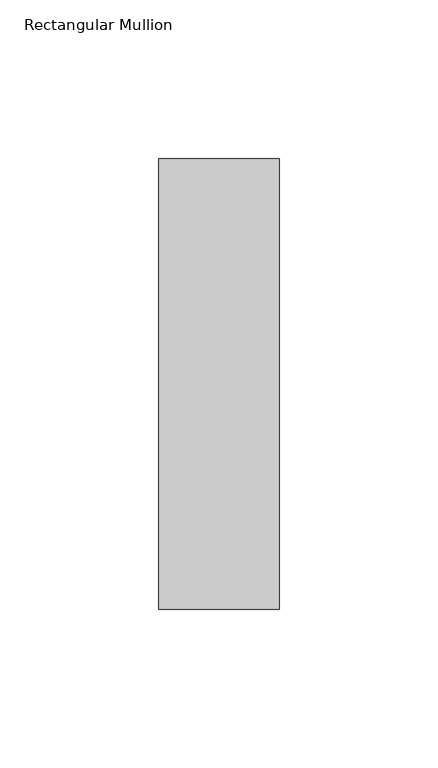
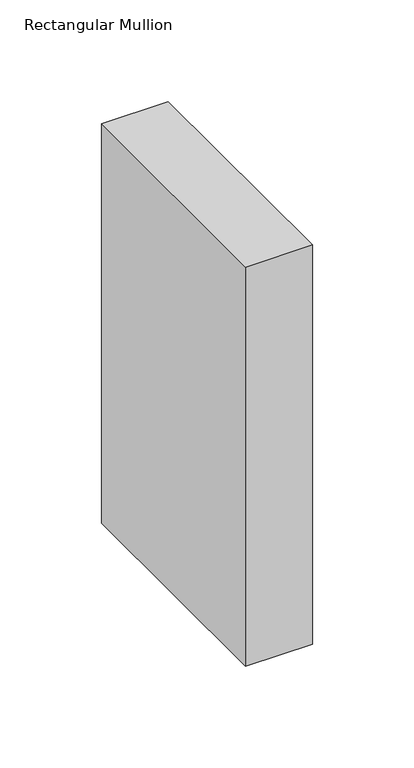
"""IFC4 building model written with IfcOpenShell, lengths in millimetres: member geometry, Rectangular Mullion : NLRS_21_CWM_hsb-regel 38x142_gen_rsf."""

from ifc_helpers import new_model, si_unit, frame, origin, place, context, project, spatial, polyline, outline, extrude, source, transform, mapped, element, save


def rectangular_mullion_5bdfe98c(model_context):
    return source(origin(), model_context, "Body", "SweptSolid", [
        extrude(outline(polyline([(19.0, -71.0), (-19.0, -71.0), (-19.0, 71.0), (19.0, 71.0), (19.0, -71.0)])), frame((0.0, 0.0, -239.8441061), z_axis=(0.0, 0.0, 1.0), x_axis=(1.0, 0.0, 0.0)), (0.0, 0.0, 1.0), 239.8441061),
    ])


if __name__ == "__main__":
    model = new_model("IFC4")
    model_context = context("Model", 3, world=origin())
    ifc_project = project(units=[si_unit("LENGTHUNIT", "METRE", prefix="MILLI")], contexts=[model_context])
    site = spatial("IfcSite", under=ifc_project)
    building = spatial("IfcBuilding", under=site)
    placement = place(None, origin())
    rectangular_mullion_shape = rectangular_mullion_5bdfe98c(model_context)
    element("IfcMember", 1, ObjectType="Rectangular Mullion : NLRS_21_CWM_hsb-regel 38x142_gen_rsf", at=placement, inside=building, context=model_context, shape_type="MappedRepresentation", body=[
        mapped(rectangular_mullion_shape, transform((0.0, 0.0, 0.0), x_axis=(1.0, 0.0, 0.0), y_axis=(0.0, 1.0, 0.0), z_axis=(0.0, 0.0, 1.0))),
    ])
    save(model, "model.ifc")

# Revit data of these elements
# Type "Rectangular Mullion : NLRS_21_CWM_hsb-regel 38x142_gen_rsf"
#   Export Type to IFC As = "IfcWall"
#   Type IfcGUID = "07M7mRoiH1CR8m_RSKIwpF"
#   Assembly Code = "21.10"
#   built-in parameter 1007322 = 0.465879 (stored number, unit not read)
#   built-in parameter 1007321 = 0.062336 (stored number, unit not read)
#   built-in parameter 1007320 = 0.062336 (stored number, unit not read)
# Element 1 (IfcMember, "Rectangular Mullion : NLRS_21_CWM_hsb-regel 38x142_gen_rsf")
#   Materials on its faces: "NLRS_i2_hout naaldhout vuren_gen_rsf"
# Materials
#   "NLRS_i2_hout naaldhout vuren_gen_rsf": class "I - Hout", colour RGB 234 199 147, transparency 0, Keynote = "i2", Manufacturer = "Revit Standards Foundation", URL = "www.revitstandards.org", Description = "hout vuren", Cost = 0
